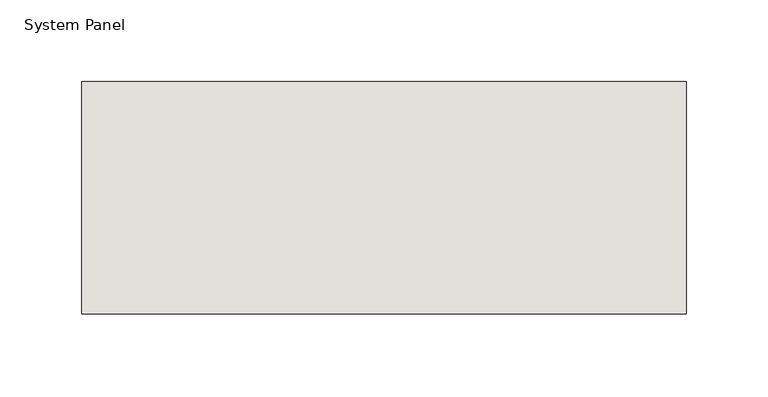
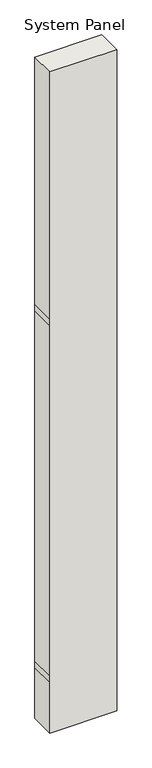
"""IFC4 building model written with IfcOpenShell, lengths in millimetres: wall geometry, System Panel : NLRS_21_CWP_hsb-vulling minerale wol 142 _gen_rsf."""

import ifcopenshell
import ifcopenshell.guid

model = None  # the IFC model being written
_history = None  # IfcOwnerHistory: only IFC2X3 demands one
_inside = {}  # id of a spatial element -> (the spatial element, [elements in it])
_under = {}  # id of a project, library or spatial element -> (it, [spatial elements below it])
_declared = {}  # id of a project -> (the project, [libraries it declares])
_typed = {}  # id of a type object -> (the type object, [elements of that type])
_made_of = {}  # id of a material, layer set ... -> (it, [elements and type objects made of it])


def new_model(schema):
    """Start an empty IFC model of exactly this schema.

    Asked for "IFC4X3", IfcOpenShell would pick the latest addendum, in which some entities
    have other attributes; the version numbers below select the first issue.
    IFC2X3 requires an IfcOwnerHistory on every rooted entity: one is made here for all.
    """
    global model, _history
    if schema == "IFC4X3":
        model = ifcopenshell.file(schema_version=(4, 3, 0, 0))
    else:
        model = ifcopenshell.file(schema=schema)
    _inside.clear()
    _under.clear()
    _declared.clear()
    _typed.clear()
    _made_of.clear()
    _history = None
    if model.schema == "IFC2X3":
        org = make("IfcOrganization", Name="unknown")
        user = make(
            "IfcPersonAndOrganization",
            ThePerson=make("IfcPerson", FamilyName="unknown"),
            TheOrganization=org,
        )
        app = make(
            "IfcApplication",
            ApplicationDeveloper=org,
            Version="unknown",
            ApplicationFullName="unknown",
            ApplicationIdentifier="unknown",
        )
        _history = make(
            "IfcOwnerHistory",
            OwningUser=user,
            OwningApplication=app,
            ChangeAction="ADDED",
            CreationDate=0,
        )
    return model


def make(cls, **values):
    """One entity of the class cls with the attributes given. An attribute that is None is left unset."""
    return model.create_entity(
        cls, **{name: value for name, value in values.items() if value is not None}
    )


def rooted(cls, **values):
    """An entity with a GlobalId (a new one), such as an element, a storey or a relation."""
    return make(cls, GlobalId=ifcopenshell.guid.new(), OwnerHistory=_history, **values)


def si_unit(unit_type, name, prefix=None):
    """IfcSIUnit, for example si_unit("LENGTHUNIT", "METRE", prefix="MILLI")."""
    return make("IfcSIUnit", UnitType=unit_type, Prefix=prefix, Name=name)


def assignment(units):
    """IfcUnitAssignment: the units of a project."""
    return None if units is None else make("IfcUnitAssignment", Units=units)


def point(xyz):
    """IfcCartesianPoint."""
    return None if xyz is None else make("IfcCartesianPoint", Coordinates=xyz)


def direction(xyz):
    """IfcDirection."""
    return None if xyz is None else make("IfcDirection", DirectionRatios=xyz)


def frame(location, z_axis=None, x_axis=None):
    """IfcAxis2Placement3D, a coordinate frame: its origin and axes. An axis left out is left unset."""
    return make(
        "IfcAxis2Placement3D",
        Location=point(location),
        Axis=direction(z_axis),
        RefDirection=direction(x_axis),
    )


def origin():
    """The frame at (0, 0, 0) with its axes left unset."""
    return frame((0.0, 0.0, 0.0))


def place(relative_to, where):
    """IfcLocalPlacement: puts the frame where relative to a parent placement (None: the world)."""
    return make(
        "IfcLocalPlacement", PlacementRelTo=relative_to, RelativePlacement=where
    )


def context(
    kind, dimensions, precision=None, world=None, true_north=None, identifier=None
):
    """IfcGeometricRepresentationContext, for example the 3D "Model" context."""
    return make(
        "IfcGeometricRepresentationContext",
        ContextIdentifier=identifier,
        ContextType=kind,
        CoordinateSpaceDimension=dimensions,
        Precision=precision,
        WorldCoordinateSystem=world,
        TrueNorth=true_north,
    )


def project(units=None, contexts=None):
    """IfcProject with its units and contexts."""
    return rooted(
        "IfcProject",
        Name="project",
        RepresentationContexts=contexts,
        UnitsInContext=assignment(units),
    )


def spatial(cls, under=None, at=None, **own):
    """A site, building, storey or space (cls), placed at a placement, below another one or the project."""
    s = rooted(cls, ObjectPlacement=at, **own)
    if under is not None:
        _under.setdefault(under.id(), (under, []))[1].append(s)
    return s


def polyline(points):
    """IfcPolyline through the points."""
    return make("IfcPolyline", Points=[point(p) for p in points])


def outline(outer, holes=None, kind="AREA"):
    """IfcArbitraryClosedProfileDef: a profile drawn as a closed curve; with holes, ...WithVoids."""
    if holes is None:
        return make("IfcArbitraryClosedProfileDef", ProfileType=kind, OuterCurve=outer)
    return make(
        "IfcArbitraryProfileDefWithVoids",
        ProfileType=kind,
        OuterCurve=outer,
        InnerCurves=holes,
    )


def extrude(swept, where, along, depth):
    """IfcExtrudedAreaSolid: the profile swept, set in the frame where, extruded along a direction by depth."""
    return make(
        "IfcExtrudedAreaSolid",
        SweptArea=swept,
        Position=where,
        ExtrudedDirection=direction(along),
        Depth=depth,
    )


def shape(context_of_items, identifier, shape_type, items):
    """IfcShapeRepresentation: the items that make up one representation, for example the "Body"."""
    return make(
        "IfcShapeRepresentation",
        ContextOfItems=context_of_items,
        RepresentationIdentifier=identifier,
        RepresentationType=shape_type,
        Items=items,
    )


def source(mapping_origin, context_of_items, identifier, shape_type, items):
    """IfcRepresentationMap: a shape defined once, which mapped items show again and again."""
    return make(
        "IfcRepresentationMap",
        MappingOrigin=mapping_origin,
        MappedRepresentation=shape(context_of_items, identifier, shape_type, items),
    )


def transform(
    local_origin,
    x_axis=None,
    y_axis=None,
    z_axis=None,
    scale=None,
    scale2=None,
    scale3=None,
    uniform=True,
):
    """IfcCartesianTransformationOperator3D, or its non-uniform kind. x_axis, y_axis, z_axis: its Axis1, 2, 3."""
    if uniform:
        return make(
            "IfcCartesianTransformationOperator3D",
            Axis1=direction(x_axis),
            Axis2=direction(y_axis),
            LocalOrigin=point(local_origin),
            Scale=scale,
            Axis3=direction(z_axis),
        )
    return make(
        "IfcCartesianTransformationOperator3DnonUniform",
        Axis1=direction(x_axis),
        Axis2=direction(y_axis),
        LocalOrigin=point(local_origin),
        Scale=scale,
        Axis3=direction(z_axis),
        Scale2=scale2,
        Scale3=scale3,
    )


def mapped(mapping_source, mapping_target):
    """IfcMappedItem: shows the shape of a source again, moved by a transform."""
    return make(
        "IfcMappedItem", MappingSource=mapping_source, MappingTarget=mapping_target
    )


def made_of(thing, what):
    """Note that an element or type object is made of a material, layer set ...; save() writes the relation."""
    if what is not None:
        _made_of.setdefault(what.id(), (what, []))[1].append(thing)
    return thing


def element(
    cls,
    number,
    at=None,
    inside=None,
    cuts=None,
    type_object=None,
    material=None,
    context=None,
    identifier="Body",
    shape_type=None,
    held_by="IfcProductDefinitionShape",
    body=None,
    shapes=None,
    **own,
):
    """One element of the class cls, such as IfcWall. Its Tag is "e" and its number.

    at: its placement. inside: the storey or other place that contains it. cuts: it is an
    opening in that element (IfcRelVoidsElement). A single representation is given by context,
    identifier, shape_type and body (its items); several are given by shapes. held_by: the class
    of the entity that holds the representations. save() writes the other relations.
    """
    e = rooted(cls, Tag="e%d" % number, ObjectPlacement=at, **own)
    if body is not None:
        shapes = [shape(context, identifier, shape_type, body)]
    if shapes is not None:
        e.Representation = make(held_by, Representations=shapes)
    if inside is not None:
        _inside.setdefault(inside.id(), (inside, []))[1].append(e)
    if cuts is not None:
        rooted(
            "IfcRelVoidsElement", RelatingBuildingElement=cuts, RelatedOpeningElement=e
        )
    if type_object is not None:
        _typed.setdefault(type_object.id(), (type_object, []))[1].append(e)
    return made_of(e, material)


def aggregate(whole, parts):
    """IfcRelAggregates: a whole, such as a stair, and the parts it consists of."""
    return rooted("IfcRelAggregates", RelatingObject=whole, RelatedObjects=parts)


def save(model, path):
    """Write the relations noted so far, then the file.

    IfcRelAggregates (storeys below a building ...), IfcRelContainedInSpatialStructure (elements
    in a storey), IfcRelDefinesByType, IfcRelAssociatesMaterial and IfcRelDeclares: one each for
    every whole, place, type object, material and project.
    """
    for whole, parts in _under.values():
        aggregate(whole, parts)
    for where, things in _inside.values():
        rooted(
            "IfcRelContainedInSpatialStructure",
            RelatedElements=things,
            RelatingStructure=where,
        )
    for kind, things in _typed.values():
        rooted("IfcRelDefinesByType", RelatedObjects=things, RelatingType=kind)
    for what, things in _made_of.values():
        rooted("IfcRelAssociatesMaterial", RelatedObjects=things, RelatingMaterial=what)
    for by, libraries in _declared.values():
        rooted("IfcRelDeclares", RelatingContext=by, RelatedDefinitions=libraries)
    model.write(path)


def system_panel_efc5a8ab(model_context):
    return source(origin(), model_context, "Body", "SweptSolid", [
        extrude(outline(polyline([(0.0, -184.5), (0.0, 184.5), (295.0, 184.5), (333.0, 184.5), (2371.0, 184.5), (2409.0, 184.5), (3849.0, 184.5), (3849.0, -184.5), (2409.0, -184.5), (2371.0, -184.5), (333.0, -184.5), (295.0, -184.5), (0.0, -184.5)])), frame((0.0, -71.0, 0.0), z_axis=(0.0, 1.0, 0.0), x_axis=(0.0, 0.0, 1.0)), (0.0, 0.0, 1.0), 142.0),
    ])


if __name__ == "__main__":
    model = new_model("IFC4")
    model_context = context("Model", 3, world=origin())
    ifc_project = project(units=[si_unit("LENGTHUNIT", "METRE", prefix="MILLI")], contexts=[model_context])
    site = spatial("IfcSite", under=ifc_project)
    building = spatial("IfcBuilding", under=site)
    placement = place(None, origin())
    system_panel_shape = system_panel_efc5a8ab(model_context)
    element("IfcWall", 1, ObjectType="System Panel : NLRS_21_CWP_hsb-vulling minerale wol 142 _gen_rsf", at=placement, inside=building, context=model_context, shape_type="MappedRepresentation", body=[
        mapped(system_panel_shape, transform((0.0, 0.0, 0.0), x_axis=(1.0, 0.0, 0.0), y_axis=(0.0, 1.0, 0.0), z_axis=(0.0, 0.0, 1.0))),
    ])
    save(model, "model.ifc")

# Revit data of these elements
# Type "System Panel : NLRS_21_CWP_hsb-vulling minerale wol 142 _gen_rsf"
#   Type IfcGUID = "07M7mRoiH1CR8m_RSKIwpC"
#   Assembly Code = "21.23"
#   IfcExportAs = "IfcWall"
# Element 1 (IfcWall, "System Panel : NLRS_21_CWP_hsb-vulling minerale wol 142 _gen_rsf")
#   Materials on its faces: "NLRS_m1_isolatie minerale wol_gen_rsf"
# Materials
#   "NLRS_m1_isolatie minerale wol_gen_rsf": class "M - Anorganische materialen", colour RGB 200 200 140, transparency 0, Keynote = "m1", Manufacturer = "Revit Standards Foundation", URL = "www.revitstandards.org", Description = "isolatie minerale wol", Cost = 0
